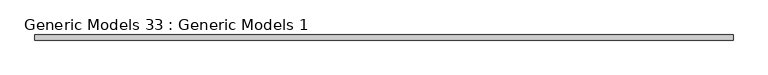
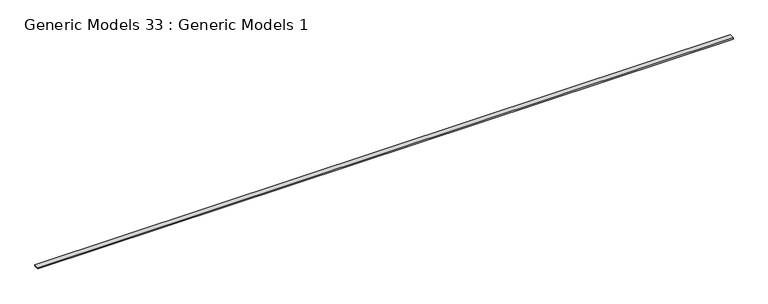
"""IFC4 building model written with IfcOpenShell, lengths in millimetres: proxy geometry, Generic Models 33 : Generic Models 1."""

from ifc_helpers import new_model, si_unit, frame, origin, place, context, project, spatial, polyline, outline, extrude, source, transform, mapped, element, save


def generic_models_33_generic_models_1_d287f3ab(model_context):
    return source(origin(), model_context, "Body", "SweptSolid", [
        extrude(outline(polyline([(-10459.9421316, 6896.3769221), (-10459.9421316, 7036.0769221), (8590.0578684, 7036.0769221), (8590.0578684, 6896.3769221), (-10459.9421316, 6896.3769221)])), frame((0.0, 0.0, 123424.696), z_axis=(0.0, 0.0, 1.0), x_axis=(1.0, 0.0, 0.0)), (0.0, 0.0, 1.0), 38.1),
    ])


if __name__ == "__main__":
    model = new_model("IFC4")
    model_context = context("Model", 3, world=origin())
    ifc_project = project(units=[si_unit("LENGTHUNIT", "METRE", prefix="MILLI")], contexts=[model_context])
    site = spatial("IfcSite", under=ifc_project)
    building = spatial("IfcBuilding", under=site)
    placement = place(None, origin())
    generic_models_33_generic_models_1_shape = generic_models_33_generic_models_1_d287f3ab(model_context)
    element("IfcBuildingElementProxy", 1, Name="Generic Models 33 : Generic Models 1", ObjectType="Generic Models 33 : Generic Models 1", at=placement, inside=building, context=model_context, shape_type="MappedRepresentation", body=[
        mapped(generic_models_33_generic_models_1_shape, transform((0.0, 0.0, 0.0), x_axis=(1.0, 0.0, 0.0), y_axis=(0.0, 1.0, 0.0), z_axis=(0.0, 0.0, 1.0))),
    ])
    save(model, "model.ifc")

# Revit data of these elements
# Element 1 (IfcBuildingElementProxy, "Generic Models 33 : Generic Models 1")
#   Materials on its faces: "_TREATED 2X BLOCKING AS REQUIRED"
# Materials
#   "_TREATED 2X BLOCKING AS REQUIRED": class "Generic", colour RGB 177 130 114, transparency 0, Cost = 0
